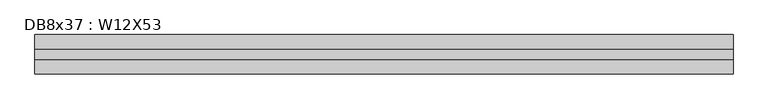
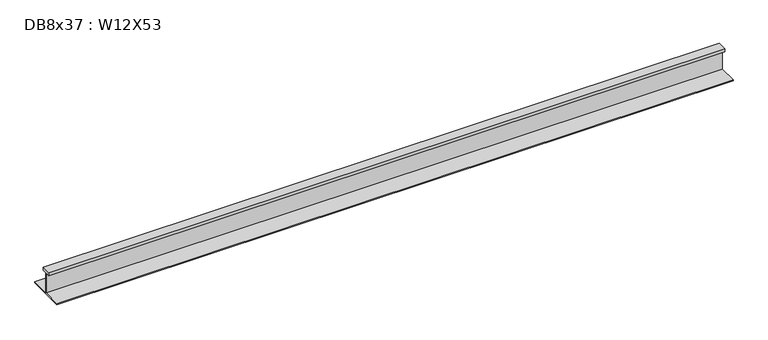
"""IFC4 building model written with IfcOpenShell, lengths in millimetres: beam geometry, DB8x37 : W12X53."""

from ifc_helpers import new_model, si_unit, frame, origin, place, context, project, spatial, polyline, outline, extrude, source, transform, mapped, element, save


def db8x37_w12x53_fe01f17b(model_context):
    return source(origin(), model_context, "Body", "SweptSolid", [
        extrude(outline(polyline([(38.1, 145.415), (38.1, 120.015), (2.921, 120.015), (2.921, -48.4505), (152.4, -48.4505), (152.4, -58.1025), (-152.4, -58.1025), (-152.4, -48.4505), (-2.921, -48.4505), (-2.921, 120.015), (-38.1, 120.015), (-38.1, 145.415), (38.1, 145.415)])), frame((-2698.3961336, 0.0, 0.0), z_axis=(1.0, 0.0, 0.0), x_axis=(0.0, 1.0, 0.0)), (0.0, 0.0, 1.0), 5394.3227218),
    ])


if __name__ == "__main__":
    model = new_model("IFC4")
    model_context = context("Model", 3, world=origin())
    ifc_project = project(units=[si_unit("LENGTHUNIT", "METRE", prefix="MILLI")], contexts=[model_context])
    site = spatial("IfcSite", under=ifc_project)
    building = spatial("IfcBuilding", under=site)
    placement = place(None, origin())
    db8x37_w12x53_shape = db8x37_w12x53_fe01f17b(model_context)
    element("IfcBeam", 1, ObjectType="DB8x37 : W12X53", at=placement, inside=building, context=model_context, shape_type="MappedRepresentation", body=[
        mapped(db8x37_w12x53_shape, transform((0.0, 0.0, 0.0), x_axis=(1.0, 0.0, 0.0), y_axis=(0.0, 1.0, 0.0), z_axis=(0.0, 0.0, 1.0))),
    ])
    save(model, "model.ifc")

# Revit data of these elements
# Type "DB8x37 : W12X53"
#   Assembly Code = "B10"
#   W = 53
#   Length [instance default] = 5' - 0"
#   bf = 0' - 10"
#   d = 1' - 0.1"
#   k = 0' - 1 3/8"
#   k2 = 0' - 0.8"
#   tf = 0' - 0.575"
#   tw = 0' - 0.345"
#   A = 0.108333 SF
#   Structural Material [instance default] = Steel ASTM A992
# Element 1 (IfcBeam, "DB8x37 : W12X53")
#   Materials on its faces: "Steel ASTM A992"
# Materials
#   "Steel ASTM A992": class "Metal", colour RGB 199 199 199, transparency 0, Description = "Structural steel 50ksi", Cost = 0
